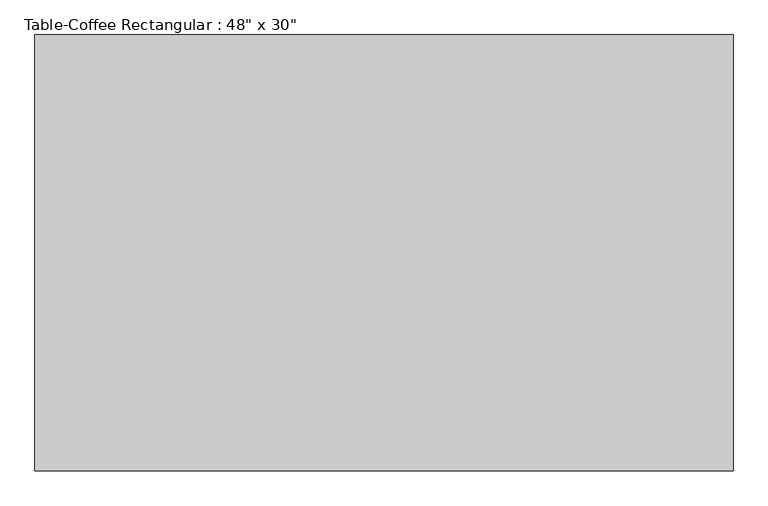
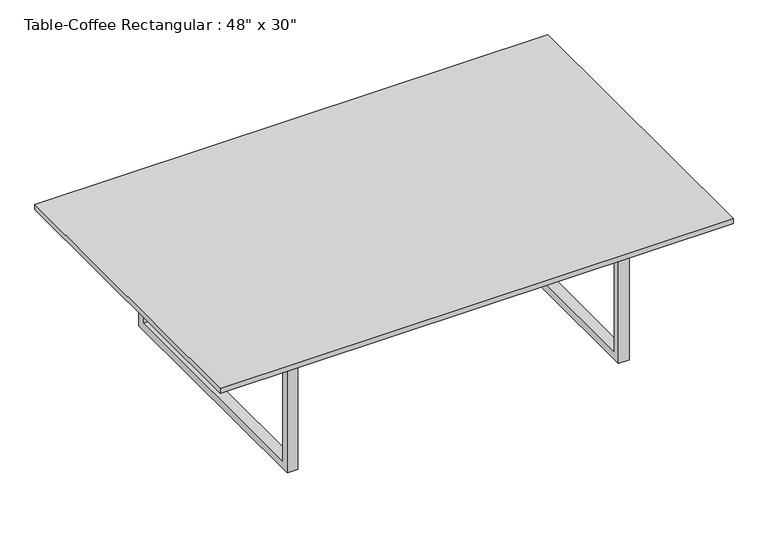
"""IFC4 building model written with IfcOpenShell, lengths in millimetres: furniture geometry."""

import ifcopenshell
import ifcopenshell.guid

model = None  # the IFC model being written
_history = None  # IfcOwnerHistory: only IFC2X3 demands one
_inside = {}  # id of a spatial element -> (the spatial element, [elements in it])
_under = {}  # id of a project, library or spatial element -> (it, [spatial elements below it])
_declared = {}  # id of a project -> (the project, [libraries it declares])
_typed = {}  # id of a type object -> (the type object, [elements of that type])
_made_of = {}  # id of a material, layer set ... -> (it, [elements and type objects made of it])


def new_model(schema):
    """Start an empty IFC model of exactly this schema.

    Asked for "IFC4X3", IfcOpenShell would pick the latest addendum, in which some entities
    have other attributes; the version numbers below select the first issue.
    IFC2X3 requires an IfcOwnerHistory on every rooted entity: one is made here for all.
    """
    global model, _history
    if schema == "IFC4X3":
        model = ifcopenshell.file(schema_version=(4, 3, 0, 0))
    else:
        model = ifcopenshell.file(schema=schema)
    _inside.clear()
    _under.clear()
    _declared.clear()
    _typed.clear()
    _made_of.clear()
    _history = None
    if model.schema == "IFC2X3":
        org = make("IfcOrganization", Name="unknown")
        user = make(
            "IfcPersonAndOrganization",
            ThePerson=make("IfcPerson", FamilyName="unknown"),
            TheOrganization=org,
        )
        app = make(
            "IfcApplication",
            ApplicationDeveloper=org,
            Version="unknown",
            ApplicationFullName="unknown",
            ApplicationIdentifier="unknown",
        )
        _history = make(
            "IfcOwnerHistory",
            OwningUser=user,
            OwningApplication=app,
            ChangeAction="ADDED",
            CreationDate=0,
        )
    return model


def make(cls, **values):
    """One entity of the class cls with the attributes given. An attribute that is None is left unset."""
    return model.create_entity(
        cls, **{name: value for name, value in values.items() if value is not None}
    )


def rooted(cls, **values):
    """An entity with a GlobalId (a new one), such as an element, a storey or a relation."""
    return make(cls, GlobalId=ifcopenshell.guid.new(), OwnerHistory=_history, **values)


def si_unit(unit_type, name, prefix=None):
    """IfcSIUnit, for example si_unit("LENGTHUNIT", "METRE", prefix="MILLI")."""
    return make("IfcSIUnit", UnitType=unit_type, Prefix=prefix, Name=name)


def assignment(units):
    """IfcUnitAssignment: the units of a project."""
    return None if units is None else make("IfcUnitAssignment", Units=units)


def point(xyz):
    """IfcCartesianPoint."""
    return None if xyz is None else make("IfcCartesianPoint", Coordinates=xyz)


def direction(xyz):
    """IfcDirection."""
    return None if xyz is None else make("IfcDirection", DirectionRatios=xyz)


def frame(location, z_axis=None, x_axis=None):
    """IfcAxis2Placement3D, a coordinate frame: its origin and axes. An axis left out is left unset."""
    return make(
        "IfcAxis2Placement3D",
        Location=point(location),
        Axis=direction(z_axis),
        RefDirection=direction(x_axis),
    )


def origin():
    """The frame at (0, 0, 0) with its axes left unset."""
    return frame((0.0, 0.0, 0.0))


def place(relative_to, where):
    """IfcLocalPlacement: puts the frame where relative to a parent placement (None: the world)."""
    return make(
        "IfcLocalPlacement", PlacementRelTo=relative_to, RelativePlacement=where
    )


def context(
    kind, dimensions, precision=None, world=None, true_north=None, identifier=None
):
    """IfcGeometricRepresentationContext, for example the 3D "Model" context."""
    return make(
        "IfcGeometricRepresentationContext",
        ContextIdentifier=identifier,
        ContextType=kind,
        CoordinateSpaceDimension=dimensions,
        Precision=precision,
        WorldCoordinateSystem=world,
        TrueNorth=true_north,
    )


def project(units=None, contexts=None):
    """IfcProject with its units and contexts."""
    return rooted(
        "IfcProject",
        Name="project",
        RepresentationContexts=contexts,
        UnitsInContext=assignment(units),
    )


def spatial(cls, under=None, at=None, **own):
    """A site, building, storey or space (cls), placed at a placement, below another one or the project."""
    s = rooted(cls, ObjectPlacement=at, **own)
    if under is not None:
        _under.setdefault(under.id(), (under, []))[1].append(s)
    return s


def polyline(points):
    """IfcPolyline through the points."""
    return make("IfcPolyline", Points=[point(p) for p in points])


def outline(outer, holes=None, kind="AREA"):
    """IfcArbitraryClosedProfileDef: a profile drawn as a closed curve; with holes, ...WithVoids."""
    if holes is None:
        return make("IfcArbitraryClosedProfileDef", ProfileType=kind, OuterCurve=outer)
    return make(
        "IfcArbitraryProfileDefWithVoids",
        ProfileType=kind,
        OuterCurve=outer,
        InnerCurves=holes,
    )


def extrude(swept, where, along, depth):
    """IfcExtrudedAreaSolid: the profile swept, set in the frame where, extruded along a direction by depth."""
    return make(
        "IfcExtrudedAreaSolid",
        SweptArea=swept,
        Position=where,
        ExtrudedDirection=direction(along),
        Depth=depth,
    )


def shape(context_of_items, identifier, shape_type, items):
    """IfcShapeRepresentation: the items that make up one representation, for example the "Body"."""
    return make(
        "IfcShapeRepresentation",
        ContextOfItems=context_of_items,
        RepresentationIdentifier=identifier,
        RepresentationType=shape_type,
        Items=items,
    )


def source(mapping_origin, context_of_items, identifier, shape_type, items):
    """IfcRepresentationMap: a shape defined once, which mapped items show again and again."""
    return make(
        "IfcRepresentationMap",
        MappingOrigin=mapping_origin,
        MappedRepresentation=shape(context_of_items, identifier, shape_type, items),
    )


def transform(
    local_origin,
    x_axis=None,
    y_axis=None,
    z_axis=None,
    scale=None,
    scale2=None,
    scale3=None,
    uniform=True,
):
    """IfcCartesianTransformationOperator3D, or its non-uniform kind. x_axis, y_axis, z_axis: its Axis1, 2, 3."""
    if uniform:
        return make(
            "IfcCartesianTransformationOperator3D",
            Axis1=direction(x_axis),
            Axis2=direction(y_axis),
            LocalOrigin=point(local_origin),
            Scale=scale,
            Axis3=direction(z_axis),
        )
    return make(
        "IfcCartesianTransformationOperator3DnonUniform",
        Axis1=direction(x_axis),
        Axis2=direction(y_axis),
        LocalOrigin=point(local_origin),
        Scale=scale,
        Axis3=direction(z_axis),
        Scale2=scale2,
        Scale3=scale3,
    )


def mapped(mapping_source, mapping_target):
    """IfcMappedItem: shows the shape of a source again, moved by a transform."""
    return make(
        "IfcMappedItem", MappingSource=mapping_source, MappingTarget=mapping_target
    )


def made_of(thing, what):
    """Note that an element or type object is made of a material, layer set ...; save() writes the relation."""
    if what is not None:
        _made_of.setdefault(what.id(), (what, []))[1].append(thing)
    return thing


def element(
    cls,
    number,
    at=None,
    inside=None,
    cuts=None,
    type_object=None,
    material=None,
    context=None,
    identifier="Body",
    shape_type=None,
    held_by="IfcProductDefinitionShape",
    body=None,
    shapes=None,
    **own,
):
    """One element of the class cls, such as IfcWall. Its Tag is "e" and its number.

    at: its placement. inside: the storey or other place that contains it. cuts: it is an
    opening in that element (IfcRelVoidsElement). A single representation is given by context,
    identifier, shape_type and body (its items); several are given by shapes. held_by: the class
    of the entity that holds the representations. save() writes the other relations.
    """
    e = rooted(cls, Tag="e%d" % number, ObjectPlacement=at, **own)
    if body is not None:
        shapes = [shape(context, identifier, shape_type, body)]
    if shapes is not None:
        e.Representation = make(held_by, Representations=shapes)
    if inside is not None:
        _inside.setdefault(inside.id(), (inside, []))[1].append(e)
    if cuts is not None:
        rooted(
            "IfcRelVoidsElement", RelatingBuildingElement=cuts, RelatedOpeningElement=e
        )
    if type_object is not None:
        _typed.setdefault(type_object.id(), (type_object, []))[1].append(e)
    return made_of(e, material)


def aggregate(whole, parts):
    """IfcRelAggregates: a whole, such as a stair, and the parts it consists of."""
    return rooted("IfcRelAggregates", RelatingObject=whole, RelatedObjects=parts)


def save(model, path):
    """Write the relations noted so far, then the file.

    IfcRelAggregates (storeys below a building ...), IfcRelContainedInSpatialStructure (elements
    in a storey), IfcRelDefinesByType, IfcRelAssociatesMaterial and IfcRelDeclares: one each for
    every whole, place, type object, material and project.
    """
    for whole, parts in _under.values():
        aggregate(whole, parts)
    for where, things in _inside.values():
        rooted(
            "IfcRelContainedInSpatialStructure",
            RelatedElements=things,
            RelatingStructure=where,
        )
    for kind, things in _typed.values():
        rooted("IfcRelDefinesByType", RelatedObjects=things, RelatingType=kind)
    for what, things in _made_of.values():
        rooted("IfcRelAssociatesMaterial", RelatedObjects=things, RelatingMaterial=what)
    for by, libraries in _declared.values():
        rooted("IfcRelDeclares", RelatingContext=by, RelatedDefinitions=libraries)
    model.write(path)


def furniture_102613a1(model_context):
    return source(origin(), model_context, "Body", "SweptSolid", [
        extrude(outline(polyline([(994.3336303, 379.1358318), (994.3336303, 360.0858318), (232.3336303, 360.0858318), (232.3336303, 379.1358318), (994.3336303, 379.1358318)])), frame((0.0, 0.0, 298.45), z_axis=(0.0, 0.0, 1.0), x_axis=(1.0, 0.0, 0.0)), (0.0, 0.0, 1.0), 19.05),
        extrude(outline(polyline([(64.8108318, 317.5), (674.4108318, 317.5), (674.4108318, 0.0), (64.8108318, 0.0), (64.8108318, 317.5)]), holes=[polyline([(83.8608318, 298.45), (83.8608318, 19.05), (655.3608318, 19.05), (655.3608318, 298.45), (83.8608318, 298.45)])]), frame((994.3336303, 0.0, 0.0), z_axis=(1.0, 0.0, 0.0), x_axis=(0.0, 1.0, 0.0)), (0.0, 0.0, 1.0), 25.4),
        extrude(outline(polyline([(64.8108318, 317.5), (674.4108318, 317.5), (674.4108318, 0.0), (64.8108318, 0.0), (64.8108318, 317.5)]), holes=[polyline([(83.8608318, 298.45), (83.8608318, 19.05), (655.3608318, 19.05), (655.3608318, 298.45), (83.8608318, 298.45)])]), frame((206.9336303, 0.0, 0.0), z_axis=(1.0, 0.0, 0.0), x_axis=(0.0, 1.0, 0.0)), (0.0, 0.0, 1.0), 25.4),
        extrude(outline(polyline([(1222.9336303, 750.6108318), (1222.9336303, -11.3891682), (3.7336303, -11.3891682), (3.7336303, 750.6108318), (1222.9336303, 750.6108318)])), frame((0.0, 0.0, 317.5), z_axis=(0.0, 0.0, 1.0), x_axis=(1.0, 0.0, 0.0)), (0.0, 0.0, 1.0), 12.7),
    ])


if __name__ == "__main__":
    model = new_model("IFC4")
    model_context = context("Model", 3, world=origin())
    ifc_project = project(units=[si_unit("LENGTHUNIT", "METRE", prefix="MILLI")], contexts=[model_context])
    site = spatial("IfcSite", under=ifc_project)
    building = spatial("IfcBuilding", under=site)
    placement = place(None, origin())
    furniture_shape = furniture_102613a1(model_context)
    element("IfcFurniture", 1, ObjectType="Table-Coffee Rectangular : 48\" x 30\"", at=placement, inside=building, context=model_context, shape_type="MappedRepresentation", body=[
        mapped(furniture_shape, transform((0.0, 0.0, 0.0), x_axis=(1.0, 0.0, 0.0), y_axis=(0.0, 1.0, 0.0), z_axis=(0.0, 0.0, 1.0))),
    ])
    save(model, "model.ifc")

# Revit data of these elements
# Type "Table-Coffee Rectangular : 48\" x 30\""
#   Assembly Code = "E2020200"
#   Height = 1' - 1"
#   Length = 4' - 0"
#   Width = 2' - 6"
#   Base Material = Metal - Chrome
#   Table Top Material = Glass - Clear, Grey
# Element 1 (IfcFurniture, "Table-Coffee Rectangular : 48\" x 30\"")
#   Materials on its faces: "Metal - Chrome", "Glass - Clear, Grey"
# Materials
#   "Metal - Chrome": class "Metal", colour RGB 244 244 244, transparency 0, Comments = "Rendering appearance not upgraded Rendering appearance not upgraded ", Description = "Chrome"
#   "Glass - Clear, Grey": class "Glass", colour RGB 252 255 255, transparency 0.64, Comments = "Rendering appearance not upgraded Rendering appearance not upgraded "
